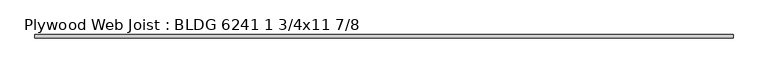
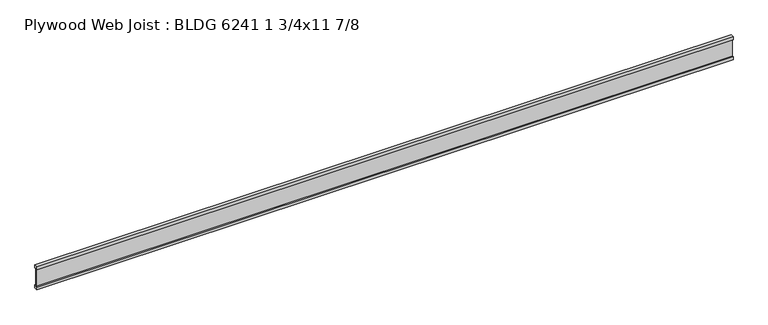
"""IFC4 building model written with IfcOpenShell, lengths in millimetres: beam geometry, Plywood Web Joist : BLDG 6241 1 3/4x11 7/8."""

from ifc_helpers import new_model, si_unit, frame, origin, place, context, project, spatial, polyline, outline, extrude, source, transform, mapped, element, save


def plywood_web_joist_bldg_6241_1_3_4x11_7_8_a6b37d20(model_context):
    return source(origin(), model_context, "Body", "SweptSolid", [
        extrude(outline(polyline([(-22.225, 150.8125), (22.225, 150.8125), (22.225, 112.7125), (4.7625, 112.7125), (4.7625, 119.0625), (-4.7625, 119.0625), (-4.7625, 112.7125), (-22.225, 112.7125), (-22.225, 150.8125)])), frame((-4330.7, 0.0, 0.0), z_axis=(1.0, 0.0, 0.0), x_axis=(0.0, 1.0, 0.0)), (0.0, 0.0, 1.0), 8661.4),
        extrude(outline(polyline([(22.225, -112.7125), (22.225, -150.8125), (-22.225, -150.8125), (-22.225, -112.7125), (-4.7625, -112.7125), (-4.7625, -118.3285374), (4.7625, -118.3285374), (4.7625, -112.7125), (22.225, -112.7125)])), frame((-4330.7, 0.0, 0.0), z_axis=(1.0, 0.0, 0.0), x_axis=(0.0, 1.0, 0.0)), (0.0, 0.0, 1.0), 8661.4),
        extrude(outline(polyline([(4330.7, 4.7625), (4330.7, -4.7625), (-4330.7, -4.7625), (-4330.7, 4.7625), (4330.7, 4.7625)])), frame((0.0, 0.0, -118.3285374), z_axis=(0.0, 0.0, 1.0), x_axis=(1.0, 0.0, 0.0)), (0.0, 0.0, 1.0), 237.3910374),
    ])


if __name__ == "__main__":
    model = new_model("IFC4")
    model_context = context("Model", 3, world=origin())
    ifc_project = project(units=[si_unit("LENGTHUNIT", "METRE", prefix="MILLI")], contexts=[model_context])
    site = spatial("IfcSite", under=ifc_project)
    building = spatial("IfcBuilding", under=site)
    placement = place(None, origin())
    plywood_web_joist_bldg_6241_1_3_4x11_7_8_shape = plywood_web_joist_bldg_6241_1_3_4x11_7_8_a6b37d20(model_context)
    element("IfcBeam", 1, ObjectType="Plywood Web Joist : BLDG 6241 1 3/4x11 7/8", at=placement, inside=building, context=model_context, shape_type="MappedRepresentation", body=[
        mapped(plywood_web_joist_bldg_6241_1_3_4x11_7_8_shape, transform((0.0, 0.0, 0.0), x_axis=(1.0, 0.0, 0.0), y_axis=(0.0, 1.0, 0.0), z_axis=(0.0, 0.0, 1.0))),
    ])
    save(model, "model.ifc")

# Revit data of these elements
# Type "Plywood Web Joist : BLDG 6241 1 3/4x11 7/8"
#   Assembly Code = "B10"
#   Length [instance default] = 5' - 0"
#   b = 0' - 1 3/4"
#   d = 0' - 11 7/8"
#   Structural Material [instance default] = Softwood, Lumber
# Element 1 (IfcBeam, "Plywood Web Joist : BLDG 6241 1 3/4x11 7/8")
#   Materials on its faces: "Softwood, Lumber"
# Materials
#   "Softwood, Lumber": class "Wood", colour RGB 223 192 134, transparency 0, Description = "Pinus Echinata", Cost = 0
